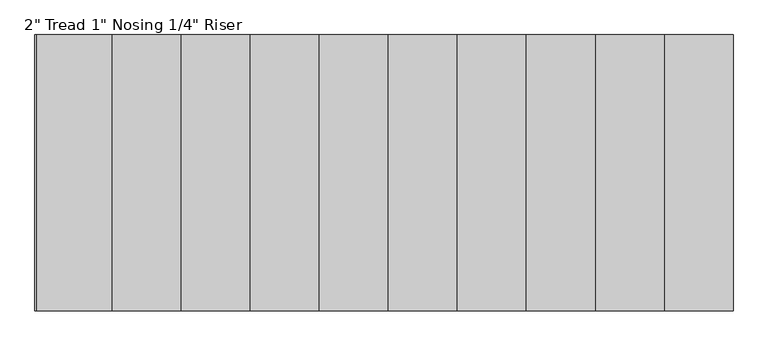
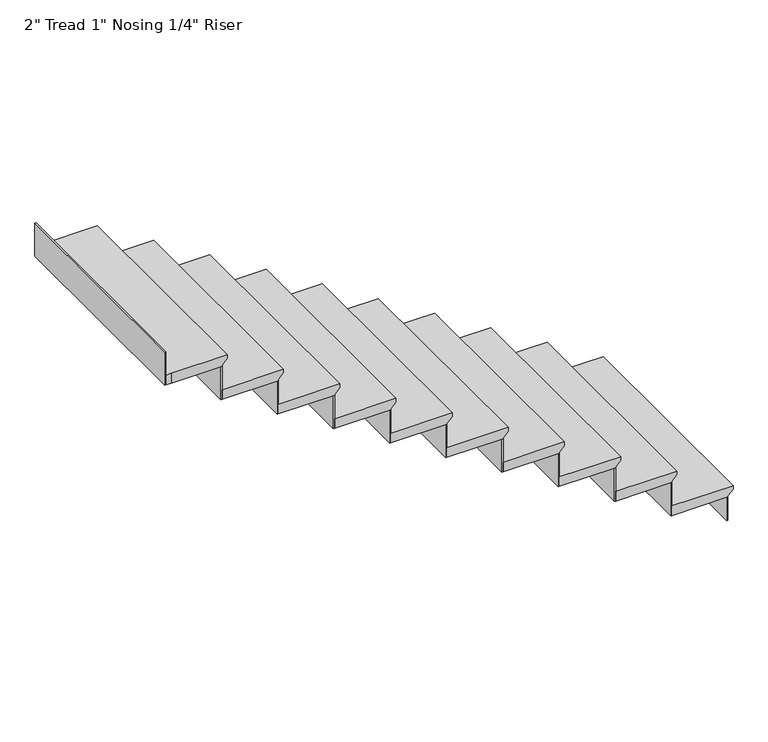
"""IFC4 building model written with IfcOpenShell, lengths in millimetres: stair flight geometry."""

from ifc_helpers import new_model, si_unit, origin, place, context, project, spatial, faceted_brep, source, transform, mapped, element, save


def stair_flight_86f709bd(model_context):
    return source(origin(), model_context, "Body", "Brep", [
        faceted_brep([(-708.6122732, 7615.1015304, 3812.7214286), (-708.6122732, 7615.1015304, 3831.7714286), (-708.6122732, 6497.5015304, 3831.7714286), (-708.6122732, 6497.5015304, 3812.7214286), (-734.0122732, 7615.1015304, 3787.3214286), (-734.0122732, 6497.5015304, 3787.3214286), (-1013.4122732, 7615.1015304, 3831.7714286), (-1013.4122732, 6497.5015304, 3831.7714286), (-734.0122732, 6497.5015304, 3780.9714286), (-1013.4122732, 6497.5015304, 3780.9714286), (-1013.4122732, 7615.1015304, 3780.9714286), (-734.0122732, 7615.1015304, 3780.9714286)], [[[0, 1, 2, 3]], [[4, 0, 3, 5]], [[2, 1, 6, 7]], [[8, 9, 10, 11]], [[2, 7, 9, 8, 5, 3]], [[8, 11, 4, 5]], [[6, 1, 0, 4, 11, 10]], [[7, 6, 10, 9]]]),
        faceted_brep([(-734.0122732, 7615.1015304, 3780.9714286), (-734.0122732, 7615.1015304, 3657.6), (-740.3622732, 7615.1015304, 3657.6), (-740.3622732, 7615.1015304, 3780.9714286), (-734.0122732, 6497.5015304, 3780.9714286), (-740.3622732, 6497.5015304, 3780.9714286), (-740.3622732, 6497.5015304, 3657.6), (-734.0122732, 6497.5015304, 3657.6)], [[[0, 1, 2, 3]], [[4, 5, 6, 7]], [[1, 0, 4, 7]], [[2, 1, 7, 6]], [[3, 2, 6, 5]], [[0, 3, 5, 4]]]),
        faceted_brep([(-1013.4122732, 7615.1015304, 3955.1428571), (-1013.4122732, 7615.1015304, 3780.9714286), (-1019.7622732, 7615.1015304, 3780.9714286), (-1019.7622732, 7615.1015304, 3955.1428571), (-1013.4122732, 6497.5015304, 3955.1428571), (-1019.7622732, 6497.5015304, 3955.1428571), (-1019.7622732, 6497.5015304, 3780.9714286), (-1013.4122732, 6497.5015304, 3780.9714286)], [[[0, 1, 2, 3]], [[4, 5, 6, 7]], [[1, 0, 4, 7]], [[2, 1, 7, 6]], [[3, 2, 6, 5]], [[0, 3, 5, 4]]]),
        faceted_brep([(-988.0122732, 6497.5015304, 4005.9428571), (-988.0122732, 7615.1015304, 4005.9428571), (-1292.8122732, 7615.1015304, 4005.9428571), (-1292.8122732, 6497.5015304, 4005.9428571), (-1013.4122732, 6497.5015304, 3955.1428571), (-1292.8122732, 6497.5015304, 3955.1428571), (-1292.8122732, 7615.1015304, 3955.1428571), (-1013.4122732, 7615.1015304, 3955.1428571), (-1013.4122732, 6497.5015304, 3961.4928571), (-988.0122732, 6497.5015304, 3986.8928571), (-1013.4122732, 7615.1015304, 3961.4928571), (-988.0122732, 7615.1015304, 3986.8928571)], [[[0, 1, 2, 3]], [[4, 5, 6, 7]], [[0, 3, 5, 4, 8, 9]], [[4, 7, 10, 8]], [[2, 1, 11, 10, 7, 6]], [[3, 2, 6, 5]], [[11, 1, 0, 9]], [[10, 11, 9, 8]]]),
        faceted_brep([(-1292.8122732, 7615.1015304, 4129.3142857), (-1292.8122732, 7615.1015304, 3955.1428571), (-1299.1622732, 7615.1015304, 3955.1428571), (-1299.1622732, 7615.1015304, 4129.3142857), (-1292.8122732, 6497.5015304, 4129.3142857), (-1299.1622732, 6497.5015304, 4129.3142857), (-1299.1622732, 6497.5015304, 3955.1428571), (-1292.8122732, 6497.5015304, 3955.1428571)], [[[0, 1, 2, 3]], [[4, 5, 6, 7]], [[1, 0, 4, 7]], [[2, 1, 7, 6]], [[3, 2, 6, 5]], [[0, 3, 5, 4]]]),
        faceted_brep([(-1267.4122732, 6497.5015304, 4180.1142857), (-1267.4122732, 7615.1015304, 4180.1142857), (-1572.2122732, 7615.1015304, 4180.1142857), (-1572.2122732, 6497.5015304, 4180.1142857), (-1292.8122732, 6497.5015304, 4129.3142857), (-1572.2122732, 6497.5015304, 4129.3142857), (-1572.2122732, 7615.1015304, 4129.3142857), (-1292.8122732, 7615.1015304, 4129.3142857), (-1292.8122732, 6497.5015304, 4135.6642857), (-1267.4122732, 6497.5015304, 4161.0642857), (-1292.8122732, 7615.1015304, 4135.6642857), (-1267.4122732, 7615.1015304, 4161.0642857)], [[[0, 1, 2, 3]], [[4, 5, 6, 7]], [[0, 3, 5, 4, 8, 9]], [[4, 7, 10, 8]], [[2, 1, 11, 10, 7, 6]], [[3, 2, 6, 5]], [[11, 1, 0, 9]], [[10, 11, 9, 8]]]),
        faceted_brep([(-1572.2122732, 7615.1015304, 4303.4857143), (-1572.2122732, 7615.1015304, 4129.3142857), (-1578.5622732, 7615.1015304, 4129.3142857), (-1578.5622732, 7615.1015304, 4303.4857143), (-1572.2122732, 6497.5015304, 4303.4857143), (-1578.5622732, 6497.5015304, 4303.4857143), (-1578.5622732, 6497.5015304, 4129.3142857), (-1572.2122732, 6497.5015304, 4129.3142857)], [[[0, 1, 2, 3]], [[4, 5, 6, 7]], [[1, 0, 4, 7]], [[2, 1, 7, 6]], [[3, 2, 6, 5]], [[0, 3, 5, 4]]]),
        faceted_brep([(-1546.8122732, 6497.5015304, 4354.2857143), (-1546.8122732, 7615.1015304, 4354.2857143), (-1851.6122732, 7615.1015304, 4354.2857143), (-1851.6122732, 6497.5015304, 4354.2857143), (-1572.2122732, 6497.5015304, 4303.4857143), (-1851.6122732, 6497.5015304, 4303.4857143), (-1851.6122732, 7615.1015304, 4303.4857143), (-1572.2122732, 7615.1015304, 4303.4857143), (-1572.2122732, 6497.5015304, 4309.8357143), (-1546.8122732, 6497.5015304, 4335.2357143), (-1572.2122732, 7615.1015304, 4309.8357143), (-1546.8122732, 7615.1015304, 4335.2357143)], [[[0, 1, 2, 3]], [[4, 5, 6, 7]], [[0, 3, 5, 4, 8, 9]], [[4, 7, 10, 8]], [[2, 1, 11, 10, 7, 6]], [[3, 2, 6, 5]], [[11, 1, 0, 9]], [[10, 11, 9, 8]]]),
        faceted_brep([(-1851.6122732, 7615.1015304, 4477.6571429), (-1851.6122732, 7615.1015304, 4303.4857143), (-1857.9622732, 7615.1015304, 4303.4857143), (-1857.9622732, 7615.1015304, 4477.6571429), (-1851.6122732, 6497.5015304, 4477.6571429), (-1857.9622732, 6497.5015304, 4477.6571429), (-1857.9622732, 6497.5015304, 4303.4857143), (-1851.6122732, 6497.5015304, 4303.4857143)], [[[0, 1, 2, 3]], [[4, 5, 6, 7]], [[1, 0, 4, 7]], [[2, 1, 7, 6]], [[3, 2, 6, 5]], [[0, 3, 5, 4]]]),
        faceted_brep([(-1826.2122732, 6497.5015304, 4528.4571429), (-1826.2122732, 7615.1015304, 4528.4571429), (-2131.0122732, 7615.1015304, 4528.4571429), (-2131.0122732, 6497.5015304, 4528.4571429), (-1851.6122732, 6497.5015304, 4477.6571429), (-2131.0122732, 6497.5015304, 4477.6571429), (-2131.0122732, 7615.1015304, 4477.6571429), (-1851.6122732, 7615.1015304, 4477.6571429), (-1851.6122732, 6497.5015304, 4484.0071429), (-1826.2122732, 6497.5015304, 4509.4071429), (-1851.6122732, 7615.1015304, 4484.0071429), (-1826.2122732, 7615.1015304, 4509.4071429)], [[[0, 1, 2, 3]], [[4, 5, 6, 7]], [[0, 3, 5, 4, 8, 9]], [[4, 7, 10, 8]], [[2, 1, 11, 10, 7, 6]], [[3, 2, 6, 5]], [[11, 1, 0, 9]], [[10, 11, 9, 8]]]),
        faceted_brep([(-2131.0122732, 7615.1015304, 4651.8285714), (-2131.0122732, 7615.1015304, 4477.6571429), (-2137.3622732, 7615.1015304, 4477.6571429), (-2137.3622732, 7615.1015304, 4651.8285714), (-2131.0122732, 6497.5015304, 4651.8285714), (-2137.3622732, 6497.5015304, 4651.8285714), (-2137.3622732, 6497.5015304, 4477.6571429), (-2131.0122732, 6497.5015304, 4477.6571429)], [[[0, 1, 2, 3]], [[4, 5, 6, 7]], [[1, 0, 4, 7]], [[2, 1, 7, 6]], [[3, 2, 6, 5]], [[0, 3, 5, 4]]]),
        faceted_brep([(-2105.6122732, 6497.5015304, 4702.6285714), (-2105.6122732, 7615.1015304, 4702.6285714), (-2410.4122732, 7615.1015304, 4702.6285714), (-2410.4122732, 6497.5015304, 4702.6285714), (-2131.0122732, 6497.5015304, 4651.8285714), (-2410.4122732, 6497.5015304, 4651.8285714), (-2410.4122732, 7615.1015304, 4651.8285714), (-2131.0122732, 7615.1015304, 4651.8285714), (-2131.0122732, 6497.5015304, 4658.1785714), (-2105.6122732, 6497.5015304, 4683.5785714), (-2131.0122732, 7615.1015304, 4658.1785714), (-2105.6122732, 7615.1015304, 4683.5785714)], [[[0, 1, 2, 3]], [[4, 5, 6, 7]], [[0, 3, 5, 4, 8, 9]], [[4, 7, 10, 8]], [[2, 1, 11, 10, 7, 6]], [[3, 2, 6, 5]], [[11, 1, 0, 9]], [[10, 11, 9, 8]]]),
        faceted_brep([(-2410.4122732, 7615.1015304, 4826.0), (-2410.4122732, 7615.1015304, 4651.8285714), (-2416.7622732, 7615.1015304, 4651.8285714), (-2416.7622732, 7615.1015304, 4826.0), (-2410.4122732, 6497.5015304, 4826.0), (-2416.7622732, 6497.5015304, 4826.0), (-2416.7622732, 6497.5015304, 4651.8285714), (-2410.4122732, 6497.5015304, 4651.8285714)], [[[0, 1, 2, 3]], [[4, 5, 6, 7]], [[1, 0, 4, 7]], [[2, 1, 7, 6]], [[3, 2, 6, 5]], [[0, 3, 5, 4]]]),
        faceted_brep([(-2385.0122732, 6497.5015304, 4876.8), (-2385.0122732, 7615.1015304, 4876.8), (-2689.8122732, 7615.1015304, 4876.8), (-2689.8122732, 6497.5015304, 4876.8), (-2410.4122732, 6497.5015304, 4826.0), (-2689.8122732, 6497.5015304, 4826.0), (-2689.8122732, 7615.1015304, 4826.0), (-2410.4122732, 7615.1015304, 4826.0), (-2410.4122732, 6497.5015304, 4832.35), (-2385.0122732, 6497.5015304, 4857.75), (-2410.4122732, 7615.1015304, 4832.35), (-2385.0122732, 7615.1015304, 4857.75)], [[[0, 1, 2, 3]], [[4, 5, 6, 7]], [[0, 3, 5, 4, 8, 9]], [[4, 7, 10, 8]], [[2, 1, 11, 10, 7, 6]], [[3, 2, 6, 5]], [[11, 1, 0, 9]], [[10, 11, 9, 8]]]),
        faceted_brep([(-2689.8122732, 7615.1015304, 5000.1714286), (-2689.8122732, 7615.1015304, 4826.0), (-2696.1622732, 7615.1015304, 4826.0), (-2696.1622732, 7615.1015304, 5000.1714286), (-2689.8122732, 6497.5015304, 5000.1714286), (-2696.1622732, 6497.5015304, 5000.1714286), (-2696.1622732, 6497.5015304, 4826.0), (-2689.8122732, 6497.5015304, 4826.0)], [[[0, 1, 2, 3]], [[4, 5, 6, 7]], [[1, 0, 4, 7]], [[2, 1, 7, 6]], [[3, 2, 6, 5]], [[0, 3, 5, 4]]]),
        faceted_brep([(-2664.4122732, 6497.5015304, 5050.9714286), (-2664.4122732, 7615.1015304, 5050.9714286), (-2969.2122732, 7615.1015304, 5050.9714286), (-2969.2122732, 6497.5015304, 5050.9714286), (-2689.8122732, 6497.5015304, 5000.1714286), (-2969.2122732, 6497.5015304, 5000.1714286), (-2969.2122732, 7615.1015304, 5000.1714286), (-2689.8122732, 7615.1015304, 5000.1714286), (-2689.8122732, 6497.5015304, 5006.5214286), (-2664.4122732, 6497.5015304, 5031.9214286), (-2689.8122732, 7615.1015304, 5006.5214286), (-2664.4122732, 7615.1015304, 5031.9214286)], [[[0, 1, 2, 3]], [[4, 5, 6, 7]], [[0, 3, 5, 4, 8, 9]], [[4, 7, 10, 8]], [[2, 1, 11, 10, 7, 6]], [[3, 2, 6, 5]], [[11, 1, 0, 9]], [[10, 11, 9, 8]]]),
        faceted_brep([(-2969.2122732, 7615.1015304, 5174.3428571), (-2969.2122732, 7615.1015304, 5000.1714286), (-2975.5622732, 7615.1015304, 5000.1714286), (-2975.5622732, 7615.1015304, 5174.3428571), (-2969.2122732, 6497.5015304, 5174.3428571), (-2975.5622732, 6497.5015304, 5174.3428571), (-2975.5622732, 6497.5015304, 5000.1714286), (-2969.2122732, 6497.5015304, 5000.1714286)], [[[0, 1, 2, 3]], [[4, 5, 6, 7]], [[1, 0, 4, 7]], [[2, 1, 7, 6]], [[3, 2, 6, 5]], [[0, 3, 5, 4]]]),
        faceted_brep([(-2943.8122732, 6497.5015304, 5225.1428571), (-2943.8122732, 7615.1015304, 5225.1428571), (-3248.6122732, 7615.1015304, 5225.1428571), (-3248.6122732, 6497.5015304, 5225.1428571), (-2969.2122732, 6497.5015304, 5174.3428571), (-3248.6122732, 6497.5015304, 5174.3428571), (-3248.6122732, 7615.1015304, 5174.3428571), (-2969.2122732, 7615.1015304, 5174.3428571), (-2969.2122732, 6497.5015304, 5180.6928571), (-2943.8122732, 6497.5015304, 5206.0928571), (-2969.2122732, 7615.1015304, 5180.6928571), (-2943.8122732, 7615.1015304, 5206.0928571)], [[[0, 1, 2, 3]], [[4, 5, 6, 7]], [[0, 3, 5, 4, 8, 9]], [[4, 7, 10, 8]], [[2, 1, 11, 10, 7, 6]], [[3, 2, 6, 5]], [[11, 1, 0, 9]], [[10, 11, 9, 8]]]),
        faceted_brep([(-3528.0122732, 7615.1015304, 5522.6857143), (-3528.0122732, 7615.1015304, 5348.5142857), (-3534.3622732, 7615.1015304, 5348.5142857), (-3534.3622732, 7615.1015304, 5522.6857143), (-3528.0122732, 6497.5015304, 5522.6857143), (-3534.3622732, 6497.5015304, 5522.6857143), (-3534.3622732, 6497.5015304, 5348.5142857), (-3528.0122732, 6497.5015304, 5348.5142857)], [[[0, 1, 2, 3]], [[4, 5, 6, 7]], [[1, 0, 4, 7]], [[2, 1, 7, 6]], [[3, 2, 6, 5]], [[0, 3, 5, 4]]]),
        faceted_brep([(-3248.6122732, 7615.1015304, 5348.5142857), (-3248.6122732, 7615.1015304, 5174.3428571), (-3254.9622732, 7615.1015304, 5174.3428571), (-3254.9622732, 7615.1015304, 5348.5142857), (-3248.6122732, 6497.5015304, 5348.5142857), (-3254.9622732, 6497.5015304, 5348.5142857), (-3254.9622732, 6497.5015304, 5174.3428571), (-3248.6122732, 6497.5015304, 5174.3428571)], [[[0, 1, 2, 3]], [[4, 5, 6, 7]], [[1, 0, 4, 7]], [[2, 1, 7, 6]], [[3, 2, 6, 5]], [[0, 3, 5, 4]]]),
        faceted_brep([(-3528.0122732, 6497.5015304, 5399.3142857), (-3502.6122732, 6497.5015304, 5399.3142857), (-3223.2122732, 6497.5015304, 5399.3142857), (-3223.2122732, 7615.1015304, 5399.3142857), (-3528.0122732, 7615.1015304, 5399.3142857), (-3502.6122732, 6497.5015304, 5348.5142857), (-3528.0122732, 6497.5015304, 5348.5142857), (-3528.0122732, 7615.1015304, 5348.5142857), (-3248.6122732, 7615.1015304, 5348.5142857), (-3248.6122732, 6497.5015304, 5348.5142857), (-3248.6122732, 6497.5015304, 5354.8642857), (-3223.2122732, 6497.5015304, 5380.2642857), (-3248.6122732, 7615.1015304, 5354.8642857), (-3223.2122732, 7615.1015304, 5380.2642857)], [[[0, 1, 2, 3, 4]], [[5, 6, 7, 8, 9]], [[1, 0, 6, 5]], [[2, 1, 5, 9, 10, 11]], [[9, 8, 12, 10]], [[4, 3, 13, 12, 8, 7]], [[0, 4, 7, 6]], [[13, 3, 2, 11]], [[12, 13, 11, 10]]]),
    ])


if __name__ == "__main__":
    model = new_model("IFC4")
    model_context = context("Model", 3, world=origin())
    ifc_project = project(units=[si_unit("LENGTHUNIT", "METRE", prefix="MILLI")], contexts=[model_context])
    site = spatial("IfcSite", under=ifc_project)
    building = spatial("IfcBuilding", under=site)
    placement = place(None, origin())
    stair_flight_shape = stair_flight_86f709bd(model_context)
    element("IfcStairFlight", 1, ObjectType="2\" Tread 1\" Nosing 1/4\" Riser", at=placement, inside=building, context=model_context, shape_type="MappedRepresentation", body=[
        mapped(stair_flight_shape, transform((0.0, 0.0, 0.0), x_axis=(1.0, 0.0, 0.0), y_axis=(0.0, 1.0, 0.0), z_axis=(0.0, 0.0, 1.0))),
    ])
    save(model, "model.ifc")
